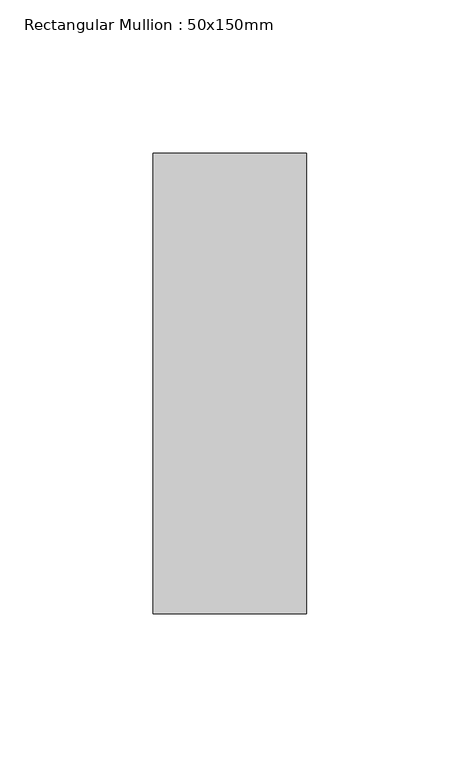
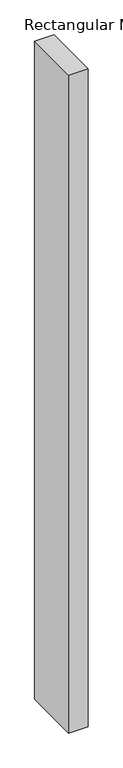
"""IFC4 building model written with IfcOpenShell, lengths in millimetres: member geometry, Rectangular Mullion : 50x150mm."""

from ifc_helpers import new_model, si_unit, frame, origin, place, context, project, spatial, polyline, outline, extrude, source, transform, mapped, element, save


def rectangular_mullion_50x150mm_ded00a16(model_context):
    return source(origin(), model_context, "Body", "SweptSolid", [
        extrude(outline(polyline([(0.0, 75.0), (0.0, -75.0), (-50.0, -75.0), (-50.0, 75.0), (0.0, 75.0)])), frame((0.0, 0.0, -1780.0), z_axis=(0.0, 0.0, 1.0), x_axis=(1.0, 0.0, 0.0)), (0.0, 0.0, 1.0), 1780.0),
    ])


if __name__ == "__main__":
    model = new_model("IFC4")
    model_context = context("Model", 3, world=origin())
    ifc_project = project(units=[si_unit("LENGTHUNIT", "METRE", prefix="MILLI")], contexts=[model_context])
    site = spatial("IfcSite", under=ifc_project)
    building = spatial("IfcBuilding", under=site)
    placement = place(None, origin())
    rectangular_mullion_50x150mm_shape = rectangular_mullion_50x150mm_ded00a16(model_context)
    element("IfcMember", 1, ObjectType="Rectangular Mullion : 50x150mm", at=placement, inside=building, context=model_context, shape_type="MappedRepresentation", body=[
        mapped(rectangular_mullion_50x150mm_shape, transform((0.0, 0.0, 0.0), x_axis=(1.0, 0.0, 0.0), y_axis=(0.0, 1.0, 0.0), z_axis=(0.0, 0.0, 1.0))),
    ])
    save(model, "model.ifc")

# Revit data of these elements
# Type "Rectangular Mullion : 50x150mm"
#   Keynote = "H11"
#   built-in parameter 1007304 = 0.492126 (stored number, unit not read)
#   built-in parameter 1007301 = 0.082021 (stored number, unit not read)
#   built-in parameter 1007300 = 0.082021 (stored number, unit not read)
# Element 1 (IfcMember, "Rectangular Mullion : 50x150mm")
#   Materials on its faces: "Aluminium"
# Materials
#   "Aluminium": class "Metal", colour RGB 247 247 247, transparency 0, Description = "Aluminium 6061", Cost = 0
